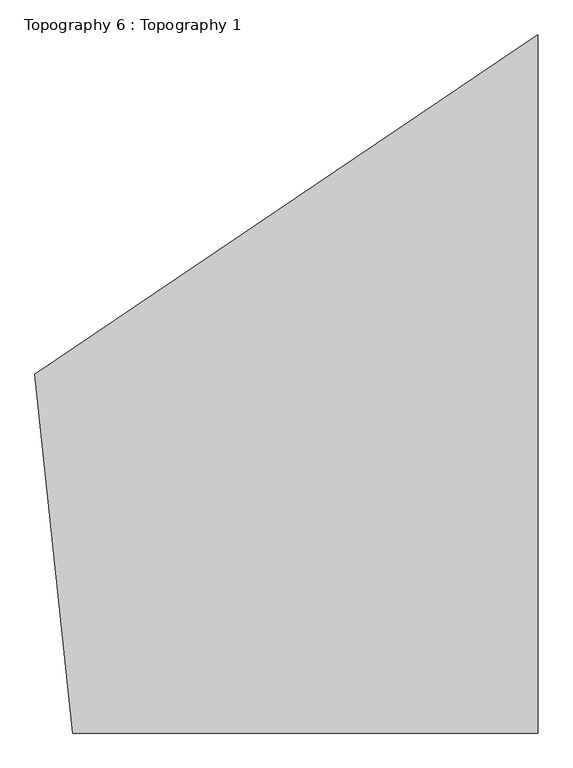
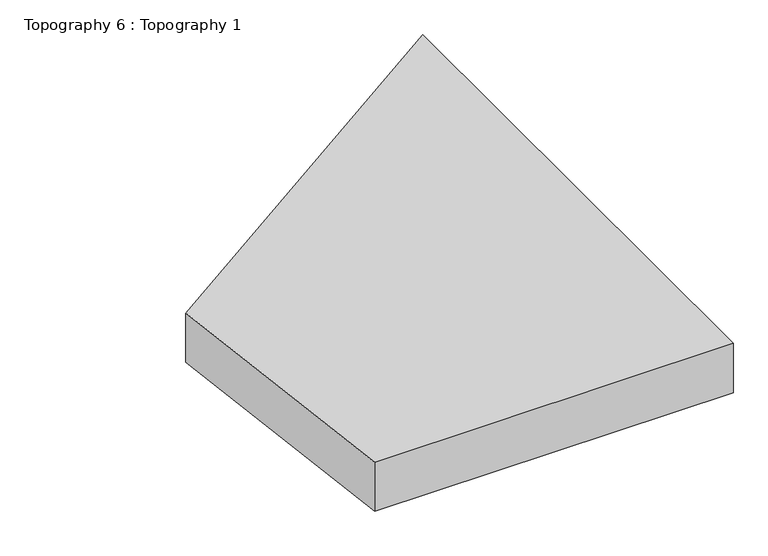
"""IFC4 building model written with IfcOpenShell, lengths in millimetres: proxy geometry, Topography 6 : Topography 1."""

from ifc_helpers import new_model, si_unit, frame, origin, place, context, project, spatial, polyline, outline, extrude, source, transform, mapped, element, save


def topography_6_topography_1_ed09c014(model_context):
    return source(origin(), model_context, "Body", "SweptSolid", [
        extrude(outline(polyline([(136325.9552311, 39054.0681482), (134220.0017656, 59090.8769425), (162308.6227529, 78036.8910248), (162308.6227529, 39054.0681482), (136325.9552311, 39054.0681482)])), frame((0.0, 0.0, -10500.0), z_axis=(0.0, 0.0, 1.0), x_axis=(1.0, 0.0, 0.0)), (0.0, 0.0, 1.0), 3770.0),
    ])


if __name__ == "__main__":
    model = new_model("IFC4")
    model_context = context("Model", 3, world=origin())
    ifc_project = project(units=[si_unit("LENGTHUNIT", "METRE", prefix="MILLI")], contexts=[model_context])
    site = spatial("IfcSite", under=ifc_project)
    building = spatial("IfcBuilding", under=site)
    placement = place(None, origin())
    topography_6_topography_1_shape = topography_6_topography_1_ed09c014(model_context)
    element("IfcBuildingElementProxy", 1, Name="Topography 6 : Topography 1", ObjectType="Topography 6 : Topography 1", at=placement, inside=building, context=model_context, shape_type="MappedRepresentation", body=[
        mapped(topography_6_topography_1_shape, transform((0.0, 0.0, 0.0), x_axis=(1.0, 0.0, 0.0), y_axis=(0.0, 1.0, 0.0), z_axis=(0.0, 0.0, 1.0))),
    ])
    save(model, "model.ifc")

# Revit data of these elements
# Element 1 (IfcBuildingElementProxy, "Topography 6 : Topography 1")
#   Materials on its faces: "Grass"
# Materials
#   "Grass": class "Generic", colour RGB 0 185 92, transparency 0, Description = "Physical material.", Cost = 0
